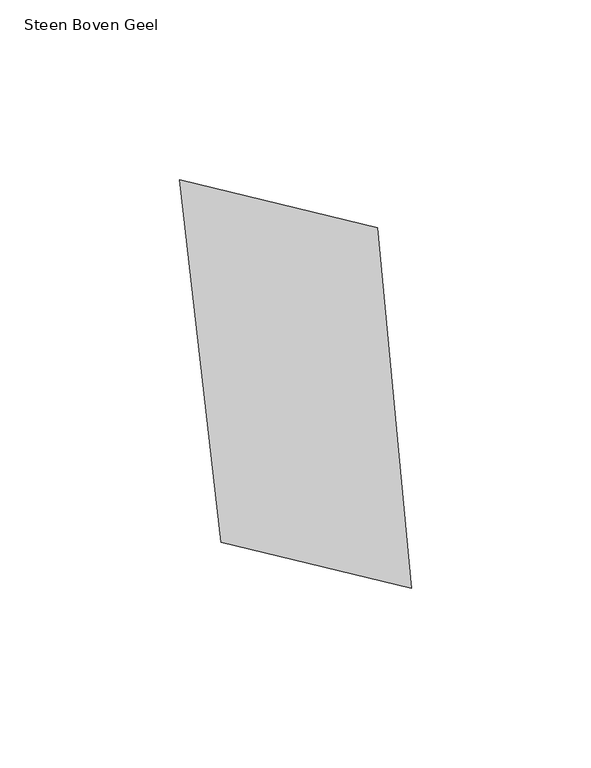
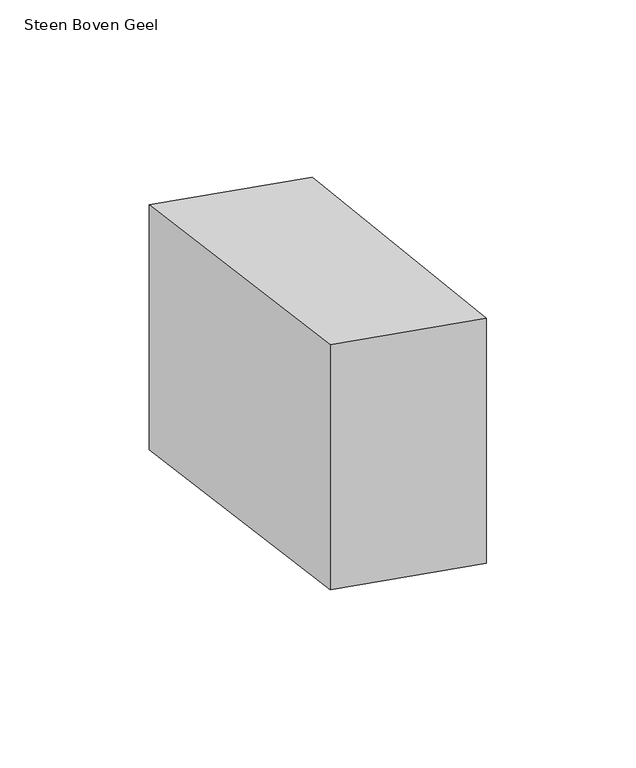
"""IFC4 building model written with IfcOpenShell, lengths in millimetres: proxy geometry, 00_GMA_steen_versie_4 : Steen Boven Geel."""

from ifc_helpers import new_model, si_unit, origin, origin_with_axes, place, context, project, spatial, polyline, outline, extrude, source, transform, mapped, element, save


def steen_boven_geel_8e220316(model_context):
    return source(origin(), model_context, "Body", "SweptSolid", [
        extrude(outline(polyline([(95.7277874, 122.422777), (105.1894721, 22.0996721), (52.1786652, 34.9130023), (40.6541305, 135.7645692), (95.7277874, 122.422777)])), origin_with_axes(), (0.0, 0.0, 1.0), 100.0),
    ])


if __name__ == "__main__":
    model = new_model("IFC4")
    model_context = context("Model", 3, world=origin())
    ifc_project = project(units=[si_unit("LENGTHUNIT", "METRE", prefix="MILLI")], contexts=[model_context])
    site = spatial("IfcSite", under=ifc_project)
    building = spatial("IfcBuilding", under=site)
    placement = place(None, origin())
    steen_boven_geel_shape = steen_boven_geel_8e220316(model_context)
    element("IfcBuildingElementProxy", 1, Name="00_GMA_steen_versie_4 : Steen Boven Geel", ObjectType="00_GMA_steen_versie_4 : Steen Boven Geel", at=placement, inside=building, context=model_context, shape_type="MappedRepresentation", body=[
        mapped(steen_boven_geel_shape, transform((0.0, 0.0, 0.0), x_axis=(1.0, 0.0, 0.0), y_axis=(0.0, 1.0, 0.0), z_axis=(0.0, 0.0, 1.0))),
    ])
    save(model, "model.ifc")

# Revit data of these elements
# Type "00_GMA_steen_versie_4 : Steen Boven Geel"
#   StootVoegHalfBoven [instance default] = 5 mm
#   StootVoegHalf [instance default] = 5 mm
#   StootVoegBreedteOnder = 10 mm
#   StootVoegBreedteBoven = 10 mm
#   Steendikte = 100 mm
#   LintVoegOnderHalf = 5 mm
#   LintVoegOnder = 10 mm
#   LintVoegBovenHalf = 0 mm
#   LintVoegBoven = 0 mm
#   materiaal = 21_steen_geel
#   MateriaalVoeg = none
#   Default Elevation = 0
# Element 1 (IfcBuildingElementProxy, "00_GMA_steen_versie_4 : Steen Boven Geel")
#   Materials on its faces: "21_steen_geel"
# Materials
#   "21_steen_geel": class "Unassigned", colour RGB 202 202 0, transparency 0, Cost = 0
